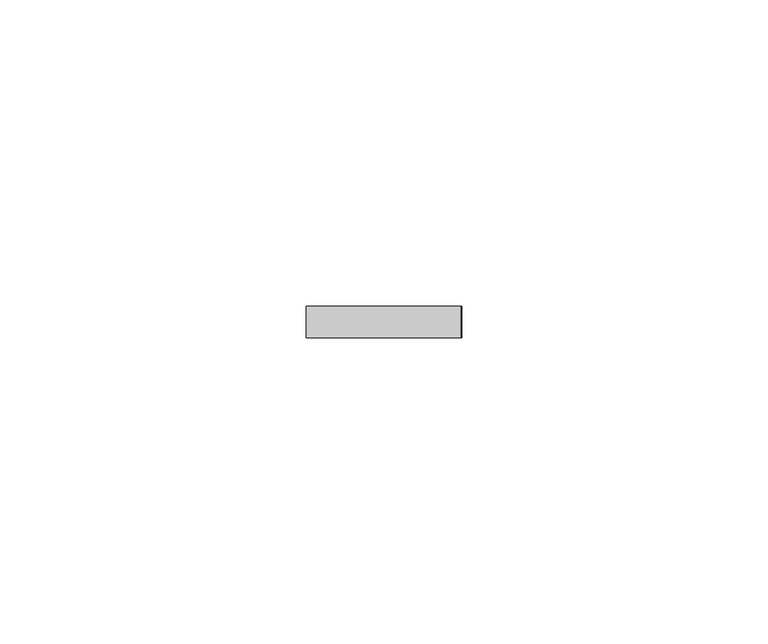
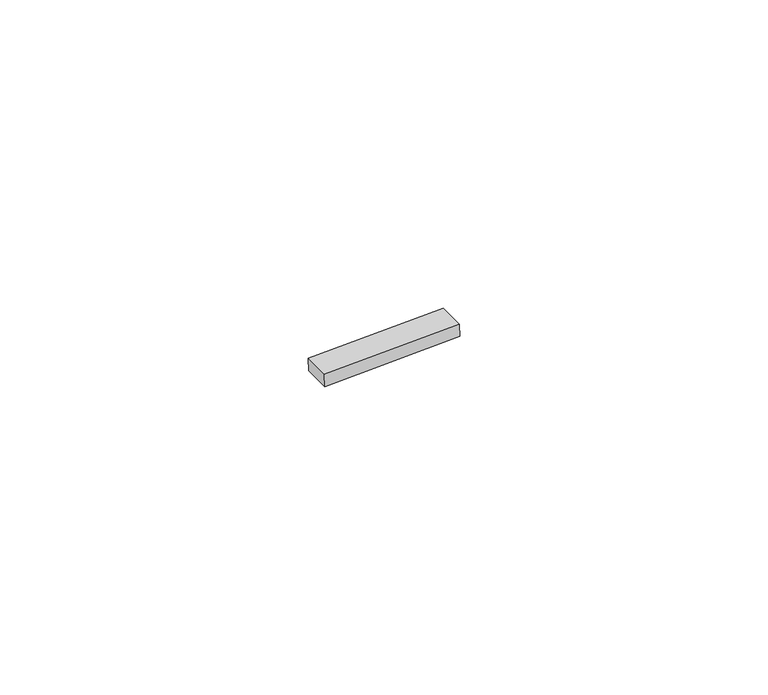
"""IFC4 building model written with IfcOpenShell, lengths in millimetres: proxy geometry, Inner panel:Inner panel:1:Inner panel:1 : Inner panel:Inner panel:300324:2:Inner panel:1:Inner panel:1 : Inner panel:Inner panel:300324:2 : Inner panel:Inner panel:1:Inner panel:1 : Inner panel:Inner panel:300324:300043:171 : Inner panel:Inner panel:1:Inner panel:1 : Inner panel:Inner panel:300324:2:Inner panel:1:Inner panel:1 : Inner panel:Inner panel:300324:2 : Inner panel:Inner panel:1:Inner panel:1 : Inner panel:Inner panel:300324:300043:308120."""

import ifcopenshell
import ifcopenshell.guid

model = None  # the IFC model being written
_history = None  # IfcOwnerHistory: only IFC2X3 demands one
_inside = {}  # id of a spatial element -> (the spatial element, [elements in it])
_under = {}  # id of a project, library or spatial element -> (it, [spatial elements below it])
_declared = {}  # id of a project -> (the project, [libraries it declares])
_typed = {}  # id of a type object -> (the type object, [elements of that type])
_made_of = {}  # id of a material, layer set ... -> (it, [elements and type objects made of it])


def new_model(schema):
    """Start an empty IFC model of exactly this schema.

    Asked for "IFC4X3", IfcOpenShell would pick the latest addendum, in which some entities
    have other attributes; the version numbers below select the first issue.
    IFC2X3 requires an IfcOwnerHistory on every rooted entity: one is made here for all.
    """
    global model, _history
    if schema == "IFC4X3":
        model = ifcopenshell.file(schema_version=(4, 3, 0, 0))
    else:
        model = ifcopenshell.file(schema=schema)
    _inside.clear()
    _under.clear()
    _declared.clear()
    _typed.clear()
    _made_of.clear()
    _history = None
    if model.schema == "IFC2X3":
        org = make("IfcOrganization", Name="unknown")
        user = make(
            "IfcPersonAndOrganization",
            ThePerson=make("IfcPerson", FamilyName="unknown"),
            TheOrganization=org,
        )
        app = make(
            "IfcApplication",
            ApplicationDeveloper=org,
            Version="unknown",
            ApplicationFullName="unknown",
            ApplicationIdentifier="unknown",
        )
        _history = make(
            "IfcOwnerHistory",
            OwningUser=user,
            OwningApplication=app,
            ChangeAction="ADDED",
            CreationDate=0,
        )
    return model


def make(cls, **values):
    """One entity of the class cls with the attributes given. An attribute that is None is left unset."""
    return model.create_entity(
        cls, **{name: value for name, value in values.items() if value is not None}
    )


def rooted(cls, **values):
    """An entity with a GlobalId (a new one), such as an element, a storey or a relation."""
    return make(cls, GlobalId=ifcopenshell.guid.new(), OwnerHistory=_history, **values)


def si_unit(unit_type, name, prefix=None):
    """IfcSIUnit, for example si_unit("LENGTHUNIT", "METRE", prefix="MILLI")."""
    return make("IfcSIUnit", UnitType=unit_type, Prefix=prefix, Name=name)


def assignment(units):
    """IfcUnitAssignment: the units of a project."""
    return None if units is None else make("IfcUnitAssignment", Units=units)


def point(xyz):
    """IfcCartesianPoint."""
    return None if xyz is None else make("IfcCartesianPoint", Coordinates=xyz)


def direction(xyz):
    """IfcDirection."""
    return None if xyz is None else make("IfcDirection", DirectionRatios=xyz)


def frame(location, z_axis=None, x_axis=None):
    """IfcAxis2Placement3D, a coordinate frame: its origin and axes. An axis left out is left unset."""
    return make(
        "IfcAxis2Placement3D",
        Location=point(location),
        Axis=direction(z_axis),
        RefDirection=direction(x_axis),
    )


def origin():
    """The frame at (0, 0, 0) with its axes left unset."""
    return frame((0.0, 0.0, 0.0))


def place(relative_to, where):
    """IfcLocalPlacement: puts the frame where relative to a parent placement (None: the world)."""
    return make(
        "IfcLocalPlacement", PlacementRelTo=relative_to, RelativePlacement=where
    )


def context(
    kind, dimensions, precision=None, world=None, true_north=None, identifier=None
):
    """IfcGeometricRepresentationContext, for example the 3D "Model" context."""
    return make(
        "IfcGeometricRepresentationContext",
        ContextIdentifier=identifier,
        ContextType=kind,
        CoordinateSpaceDimension=dimensions,
        Precision=precision,
        WorldCoordinateSystem=world,
        TrueNorth=true_north,
    )


def project(units=None, contexts=None):
    """IfcProject with its units and contexts."""
    return rooted(
        "IfcProject",
        Name="project",
        RepresentationContexts=contexts,
        UnitsInContext=assignment(units),
    )


def spatial(cls, under=None, at=None, **own):
    """A site, building, storey or space (cls), placed at a placement, below another one or the project."""
    s = rooted(cls, ObjectPlacement=at, **own)
    if under is not None:
        _under.setdefault(under.id(), (under, []))[1].append(s)
    return s


def polyline(points):
    """IfcPolyline through the points."""
    return make("IfcPolyline", Points=[point(p) for p in points])


def outline(outer, holes=None, kind="AREA"):
    """IfcArbitraryClosedProfileDef: a profile drawn as a closed curve; with holes, ...WithVoids."""
    if holes is None:
        return make("IfcArbitraryClosedProfileDef", ProfileType=kind, OuterCurve=outer)
    return make(
        "IfcArbitraryProfileDefWithVoids",
        ProfileType=kind,
        OuterCurve=outer,
        InnerCurves=holes,
    )


def extrude(swept, where, along, depth):
    """IfcExtrudedAreaSolid: the profile swept, set in the frame where, extruded along a direction by depth."""
    return make(
        "IfcExtrudedAreaSolid",
        SweptArea=swept,
        Position=where,
        ExtrudedDirection=direction(along),
        Depth=depth,
    )


def shape(context_of_items, identifier, shape_type, items):
    """IfcShapeRepresentation: the items that make up one representation, for example the "Body"."""
    return make(
        "IfcShapeRepresentation",
        ContextOfItems=context_of_items,
        RepresentationIdentifier=identifier,
        RepresentationType=shape_type,
        Items=items,
    )


def source(mapping_origin, context_of_items, identifier, shape_type, items):
    """IfcRepresentationMap: a shape defined once, which mapped items show again and again."""
    return make(
        "IfcRepresentationMap",
        MappingOrigin=mapping_origin,
        MappedRepresentation=shape(context_of_items, identifier, shape_type, items),
    )


def transform(
    local_origin,
    x_axis=None,
    y_axis=None,
    z_axis=None,
    scale=None,
    scale2=None,
    scale3=None,
    uniform=True,
):
    """IfcCartesianTransformationOperator3D, or its non-uniform kind. x_axis, y_axis, z_axis: its Axis1, 2, 3."""
    if uniform:
        return make(
            "IfcCartesianTransformationOperator3D",
            Axis1=direction(x_axis),
            Axis2=direction(y_axis),
            LocalOrigin=point(local_origin),
            Scale=scale,
            Axis3=direction(z_axis),
        )
    return make(
        "IfcCartesianTransformationOperator3DnonUniform",
        Axis1=direction(x_axis),
        Axis2=direction(y_axis),
        LocalOrigin=point(local_origin),
        Scale=scale,
        Axis3=direction(z_axis),
        Scale2=scale2,
        Scale3=scale3,
    )


def mapped(mapping_source, mapping_target):
    """IfcMappedItem: shows the shape of a source again, moved by a transform."""
    return make(
        "IfcMappedItem", MappingSource=mapping_source, MappingTarget=mapping_target
    )


def made_of(thing, what):
    """Note that an element or type object is made of a material, layer set ...; save() writes the relation."""
    if what is not None:
        _made_of.setdefault(what.id(), (what, []))[1].append(thing)
    return thing


def element(
    cls,
    number,
    at=None,
    inside=None,
    cuts=None,
    type_object=None,
    material=None,
    context=None,
    identifier="Body",
    shape_type=None,
    held_by="IfcProductDefinitionShape",
    body=None,
    shapes=None,
    **own,
):
    """One element of the class cls, such as IfcWall. Its Tag is "e" and its number.

    at: its placement. inside: the storey or other place that contains it. cuts: it is an
    opening in that element (IfcRelVoidsElement). A single representation is given by context,
    identifier, shape_type and body (its items); several are given by shapes. held_by: the class
    of the entity that holds the representations. save() writes the other relations.
    """
    e = rooted(cls, Tag="e%d" % number, ObjectPlacement=at, **own)
    if body is not None:
        shapes = [shape(context, identifier, shape_type, body)]
    if shapes is not None:
        e.Representation = make(held_by, Representations=shapes)
    if inside is not None:
        _inside.setdefault(inside.id(), (inside, []))[1].append(e)
    if cuts is not None:
        rooted(
            "IfcRelVoidsElement", RelatingBuildingElement=cuts, RelatedOpeningElement=e
        )
    if type_object is not None:
        _typed.setdefault(type_object.id(), (type_object, []))[1].append(e)
    return made_of(e, material)


def aggregate(whole, parts):
    """IfcRelAggregates: a whole, such as a stair, and the parts it consists of."""
    return rooted("IfcRelAggregates", RelatingObject=whole, RelatedObjects=parts)


def save(model, path):
    """Write the relations noted so far, then the file.

    IfcRelAggregates (storeys below a building ...), IfcRelContainedInSpatialStructure (elements
    in a storey), IfcRelDefinesByType, IfcRelAssociatesMaterial and IfcRelDeclares: one each for
    every whole, place, type object, material and project.
    """
    for whole, parts in _under.values():
        aggregate(whole, parts)
    for where, things in _inside.values():
        rooted(
            "IfcRelContainedInSpatialStructure",
            RelatedElements=things,
            RelatingStructure=where,
        )
    for kind, things in _typed.values():
        rooted("IfcRelDefinesByType", RelatedObjects=things, RelatingType=kind)
    for what, things in _made_of.values():
        rooted("IfcRelAssociatesMaterial", RelatedObjects=things, RelatingMaterial=what)
    for by, libraries in _declared.values():
        rooted("IfcRelDeclares", RelatingContext=by, RelatedDefinitions=libraries)
    model.write(path)


def generic_models_66c0dd8a(model_context):
    return source(origin(), model_context, "Body", "SweptSolid", [
        extrude(outline(polyline([(0.0, -25.4), (0.0, 0.0), (5.213809, 0.0), (5.213809, -25.4), (0.0, -25.4)])), frame((560380.9331581, -564181.307991, 3950.5346612), z_axis=(-0.041630544712223896, 0.0, 0.9991330730923502), x_axis=(0.0, -1.0, 0.0)), (0.0, 0.0, 1.0), 2.4763745),
    ])


if __name__ == "__main__":
    model = new_model("IFC4")
    model_context = context("Model", 3, world=origin())
    ifc_project = project(units=[si_unit("LENGTHUNIT", "METRE", prefix="MILLI")], contexts=[model_context])
    site = spatial("IfcSite", under=ifc_project)
    building = spatial("IfcBuilding", under=site)
    placement = place(None, origin())
    generic_models_shape = generic_models_66c0dd8a(model_context)
    element("IfcBuildingElementProxy", 1, Name="Inner panel:Inner panel:1:Inner panel:1 : Inner panel:Inner panel:300324:2:Inner panel:1:Inner panel:1 : Inner panel:Inner panel:300324:2 : Inner panel:Inner panel:1:Inner panel:1 : Inner panel:Inner panel:300324:300043:171 : Inner panel:Inner panel:1:Inner panel:1 : Inner panel:Inner panel:300324:2:Inner panel:1:Inner panel:1 : Inner panel:Inner panel:300324:2 : Inner panel:Inner panel:1:Inner panel:1 : Inner panel:Inner panel:300324:300043:308120", ObjectType="Inner panel:Inner panel:1:Inner panel:1 : Inner panel:Inner panel:300324:2:Inner panel:1:Inner panel:1 : Inner panel:Inner panel:300324:2 : Inner panel:Inner panel:1:Inner panel:1 : Inner panel:Inner panel:300324:300043:171 : Inner panel:Inner panel:1:Inner panel:1 : Inner panel:Inner panel:300324:2:Inner panel:1:Inner panel:1 : Inner panel:Inner panel:300324:2 : Inner panel:Inner panel:1:Inner panel:1 : Inner panel:Inner panel:300324:300043:308120", at=placement, inside=building, context=model_context, shape_type="MappedRepresentation", body=[
        mapped(generic_models_shape, transform((0.0, 0.0, 0.0), x_axis=(1.0, 0.0, 0.0), y_axis=(0.0, 1.0, 0.0), z_axis=(0.0, 0.0, 1.0))),
    ])
    save(model, "model.ifc")

# Revit data of these elements
# Type "Inner panel:Inner panel:1:Inner panel:1 : Inner panel:Inner panel:300324:2:Inner panel:1:Inner panel:1 : Inner panel:Inner panel:300324:2 : Inner panel:Inner panel:1:Inner panel:1 : Inner panel:Inner panel:300324:300043:171 : Inner panel:Inner panel:1:Inner panel:1 : Inner panel:Inner panel:300324:2:Inner panel:1:Inner panel:1 : Inner panel:Inner panel:300324:2 : Inner panel:Inner panel:1:Inner panel:1 : Inner panel:Inner panel:300324:300043:308120"
#   NameOverride = "Inner panel:Inner panel:1:Inner panel:1 : Inner panel:Inner panel:300324:2:Inner panel:1:Inner panel:1 : Inner panel:Inner panel:300324:2 : Inner panel:Inner panel:1:Inner panel:1 : Inner panel:Inner panel:300324:300043:308120"
#   ObjectTypeOverride = "Inner panel:1:Inner panel:1 : Inner panel:Inner panel:300324:2 : Inner panel:Inner panel:1:Inner panel:1 : Inner panel:Inner panel:300324:300043"
#   Reference = "Inner panel"
#   Tag = "308120"
# Element 1 (IfcBuildingElementProxy, "Inner panel:Inner panel:1:Inner panel:1 : Inner panel:Inner panel:300324:2:Inner panel:1:Inner panel:1 : Inner panel:Inner panel:300324:2 : Inner panel:Inner panel:1:Inner panel:1 : Inner panel:Inner panel:300324:300043:171 : Inner panel:Inner panel:1:Inner panel:1 : Inner panel:Inner panel:300324:2:Inner panel:1:Inner panel:1 : Inner panel:Inner panel:300324:2 : Inner panel:Inner panel:1:Inner panel:1 : Inner panel:Inner panel:300324:300043:308120")
#   Materials on its faces: "AT CLIP - 1\" WIDE NON ABSORBENT, WEATHER-RESISTANT NEOPRENE/EPDM/SBR FOAM"
# Materials
#   "AT CLIP - 1\" WIDE NON ABSORBENT, WEATHER-RESISTANT NEOPRENE/EPDM/SBR FOAM": class "Generic", colour RGB 85 85 85, transparency 0, Cost = 0
